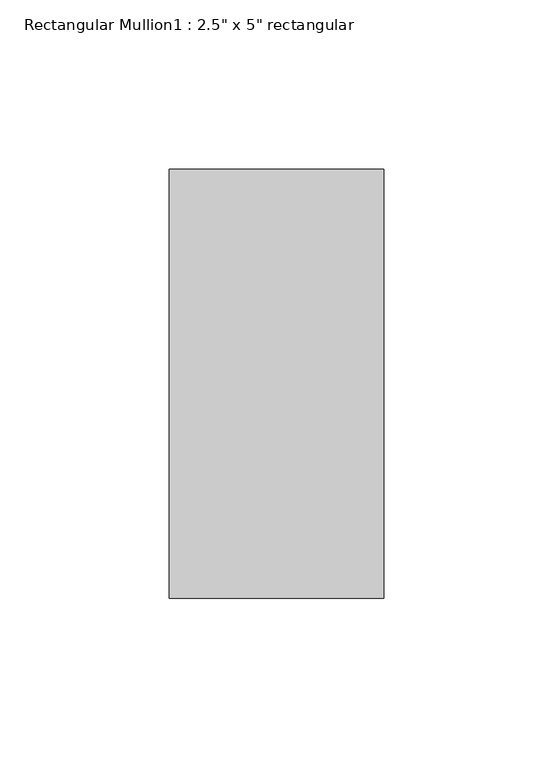
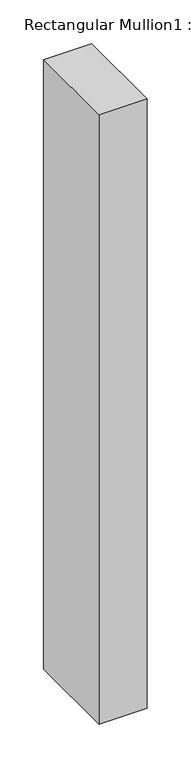
"""IFC4 building model written with IfcOpenShell, lengths in millimetres: member geometry."""

import ifcopenshell
import ifcopenshell.guid

model = None  # the IFC model being written
_history = None  # IfcOwnerHistory: only IFC2X3 demands one
_inside = {}  # id of a spatial element -> (the spatial element, [elements in it])
_under = {}  # id of a project, library or spatial element -> (it, [spatial elements below it])
_declared = {}  # id of a project -> (the project, [libraries it declares])
_typed = {}  # id of a type object -> (the type object, [elements of that type])
_made_of = {}  # id of a material, layer set ... -> (it, [elements and type objects made of it])


def new_model(schema):
    """Start an empty IFC model of exactly this schema.

    Asked for "IFC4X3", IfcOpenShell would pick the latest addendum, in which some entities
    have other attributes; the version numbers below select the first issue.
    IFC2X3 requires an IfcOwnerHistory on every rooted entity: one is made here for all.
    """
    global model, _history
    if schema == "IFC4X3":
        model = ifcopenshell.file(schema_version=(4, 3, 0, 0))
    else:
        model = ifcopenshell.file(schema=schema)
    _inside.clear()
    _under.clear()
    _declared.clear()
    _typed.clear()
    _made_of.clear()
    _history = None
    if model.schema == "IFC2X3":
        org = make("IfcOrganization", Name="unknown")
        user = make(
            "IfcPersonAndOrganization",
            ThePerson=make("IfcPerson", FamilyName="unknown"),
            TheOrganization=org,
        )
        app = make(
            "IfcApplication",
            ApplicationDeveloper=org,
            Version="unknown",
            ApplicationFullName="unknown",
            ApplicationIdentifier="unknown",
        )
        _history = make(
            "IfcOwnerHistory",
            OwningUser=user,
            OwningApplication=app,
            ChangeAction="ADDED",
            CreationDate=0,
        )
    return model


def make(cls, **values):
    """One entity of the class cls with the attributes given. An attribute that is None is left unset."""
    return model.create_entity(
        cls, **{name: value for name, value in values.items() if value is not None}
    )


def rooted(cls, **values):
    """An entity with a GlobalId (a new one), such as an element, a storey or a relation."""
    return make(cls, GlobalId=ifcopenshell.guid.new(), OwnerHistory=_history, **values)


def si_unit(unit_type, name, prefix=None):
    """IfcSIUnit, for example si_unit("LENGTHUNIT", "METRE", prefix="MILLI")."""
    return make("IfcSIUnit", UnitType=unit_type, Prefix=prefix, Name=name)


def assignment(units):
    """IfcUnitAssignment: the units of a project."""
    return None if units is None else make("IfcUnitAssignment", Units=units)


def point(xyz):
    """IfcCartesianPoint."""
    return None if xyz is None else make("IfcCartesianPoint", Coordinates=xyz)


def direction(xyz):
    """IfcDirection."""
    return None if xyz is None else make("IfcDirection", DirectionRatios=xyz)


def frame(location, z_axis=None, x_axis=None):
    """IfcAxis2Placement3D, a coordinate frame: its origin and axes. An axis left out is left unset."""
    return make(
        "IfcAxis2Placement3D",
        Location=point(location),
        Axis=direction(z_axis),
        RefDirection=direction(x_axis),
    )


def origin():
    """The frame at (0, 0, 0) with its axes left unset."""
    return frame((0.0, 0.0, 0.0))


def place(relative_to, where):
    """IfcLocalPlacement: puts the frame where relative to a parent placement (None: the world)."""
    return make(
        "IfcLocalPlacement", PlacementRelTo=relative_to, RelativePlacement=where
    )


def context(
    kind, dimensions, precision=None, world=None, true_north=None, identifier=None
):
    """IfcGeometricRepresentationContext, for example the 3D "Model" context."""
    return make(
        "IfcGeometricRepresentationContext",
        ContextIdentifier=identifier,
        ContextType=kind,
        CoordinateSpaceDimension=dimensions,
        Precision=precision,
        WorldCoordinateSystem=world,
        TrueNorth=true_north,
    )


def project(units=None, contexts=None):
    """IfcProject with its units and contexts."""
    return rooted(
        "IfcProject",
        Name="project",
        RepresentationContexts=contexts,
        UnitsInContext=assignment(units),
    )


def spatial(cls, under=None, at=None, **own):
    """A site, building, storey or space (cls), placed at a placement, below another one or the project."""
    s = rooted(cls, ObjectPlacement=at, **own)
    if under is not None:
        _under.setdefault(under.id(), (under, []))[1].append(s)
    return s


def polyline(points):
    """IfcPolyline through the points."""
    return make("IfcPolyline", Points=[point(p) for p in points])


def outline(outer, holes=None, kind="AREA"):
    """IfcArbitraryClosedProfileDef: a profile drawn as a closed curve; with holes, ...WithVoids."""
    if holes is None:
        return make("IfcArbitraryClosedProfileDef", ProfileType=kind, OuterCurve=outer)
    return make(
        "IfcArbitraryProfileDefWithVoids",
        ProfileType=kind,
        OuterCurve=outer,
        InnerCurves=holes,
    )


def extrude(swept, where, along, depth):
    """IfcExtrudedAreaSolid: the profile swept, set in the frame where, extruded along a direction by depth."""
    return make(
        "IfcExtrudedAreaSolid",
        SweptArea=swept,
        Position=where,
        ExtrudedDirection=direction(along),
        Depth=depth,
    )


def shape(context_of_items, identifier, shape_type, items):
    """IfcShapeRepresentation: the items that make up one representation, for example the "Body"."""
    return make(
        "IfcShapeRepresentation",
        ContextOfItems=context_of_items,
        RepresentationIdentifier=identifier,
        RepresentationType=shape_type,
        Items=items,
    )


def source(mapping_origin, context_of_items, identifier, shape_type, items):
    """IfcRepresentationMap: a shape defined once, which mapped items show again and again."""
    return make(
        "IfcRepresentationMap",
        MappingOrigin=mapping_origin,
        MappedRepresentation=shape(context_of_items, identifier, shape_type, items),
    )


def transform(
    local_origin,
    x_axis=None,
    y_axis=None,
    z_axis=None,
    scale=None,
    scale2=None,
    scale3=None,
    uniform=True,
):
    """IfcCartesianTransformationOperator3D, or its non-uniform kind. x_axis, y_axis, z_axis: its Axis1, 2, 3."""
    if uniform:
        return make(
            "IfcCartesianTransformationOperator3D",
            Axis1=direction(x_axis),
            Axis2=direction(y_axis),
            LocalOrigin=point(local_origin),
            Scale=scale,
            Axis3=direction(z_axis),
        )
    return make(
        "IfcCartesianTransformationOperator3DnonUniform",
        Axis1=direction(x_axis),
        Axis2=direction(y_axis),
        LocalOrigin=point(local_origin),
        Scale=scale,
        Axis3=direction(z_axis),
        Scale2=scale2,
        Scale3=scale3,
    )


def mapped(mapping_source, mapping_target):
    """IfcMappedItem: shows the shape of a source again, moved by a transform."""
    return make(
        "IfcMappedItem", MappingSource=mapping_source, MappingTarget=mapping_target
    )


def made_of(thing, what):
    """Note that an element or type object is made of a material, layer set ...; save() writes the relation."""
    if what is not None:
        _made_of.setdefault(what.id(), (what, []))[1].append(thing)
    return thing


def element(
    cls,
    number,
    at=None,
    inside=None,
    cuts=None,
    type_object=None,
    material=None,
    context=None,
    identifier="Body",
    shape_type=None,
    held_by="IfcProductDefinitionShape",
    body=None,
    shapes=None,
    **own,
):
    """One element of the class cls, such as IfcWall. Its Tag is "e" and its number.

    at: its placement. inside: the storey or other place that contains it. cuts: it is an
    opening in that element (IfcRelVoidsElement). A single representation is given by context,
    identifier, shape_type and body (its items); several are given by shapes. held_by: the class
    of the entity that holds the representations. save() writes the other relations.
    """
    e = rooted(cls, Tag="e%d" % number, ObjectPlacement=at, **own)
    if body is not None:
        shapes = [shape(context, identifier, shape_type, body)]
    if shapes is not None:
        e.Representation = make(held_by, Representations=shapes)
    if inside is not None:
        _inside.setdefault(inside.id(), (inside, []))[1].append(e)
    if cuts is not None:
        rooted(
            "IfcRelVoidsElement", RelatingBuildingElement=cuts, RelatedOpeningElement=e
        )
    if type_object is not None:
        _typed.setdefault(type_object.id(), (type_object, []))[1].append(e)
    return made_of(e, material)


def aggregate(whole, parts):
    """IfcRelAggregates: a whole, such as a stair, and the parts it consists of."""
    return rooted("IfcRelAggregates", RelatingObject=whole, RelatedObjects=parts)


def save(model, path):
    """Write the relations noted so far, then the file.

    IfcRelAggregates (storeys below a building ...), IfcRelContainedInSpatialStructure (elements
    in a storey), IfcRelDefinesByType, IfcRelAssociatesMaterial and IfcRelDeclares: one each for
    every whole, place, type object, material and project.
    """
    for whole, parts in _under.values():
        aggregate(whole, parts)
    for where, things in _inside.values():
        rooted(
            "IfcRelContainedInSpatialStructure",
            RelatedElements=things,
            RelatingStructure=where,
        )
    for kind, things in _typed.values():
        rooted("IfcRelDefinesByType", RelatedObjects=things, RelatingType=kind)
    for what, things in _made_of.values():
        rooted("IfcRelAssociatesMaterial", RelatedObjects=things, RelatingMaterial=what)
    for by, libraries in _declared.values():
        rooted("IfcRelDeclares", RelatingContext=by, RelatedDefinitions=libraries)
    model.write(path)


def member_d2e7e466(model_context):
    return source(origin(), model_context, "Body", "SweptSolid", [
        extrude(outline(polyline([(0.0, 63.5), (0.0, -63.5), (-63.5, -63.5), (-63.5, 63.5), (0.0, 63.5)])), frame((0.0, 0.0, -850.9), z_axis=(0.0, 0.0, 1.0), x_axis=(1.0, 0.0, 0.0)), (0.0, 0.0, 1.0), 850.9),
    ])


if __name__ == "__main__":
    model = new_model("IFC4")
    model_context = context("Model", 3, world=origin())
    ifc_project = project(units=[si_unit("LENGTHUNIT", "METRE", prefix="MILLI")], contexts=[model_context])
    site = spatial("IfcSite", under=ifc_project)
    building = spatial("IfcBuilding", under=site)
    placement = place(None, origin())
    member_shape = member_d2e7e466(model_context)
    element("IfcMember", 1, ObjectType="Rectangular Mullion1 : 2.5\" x 5\" rectangular", at=placement, inside=building, context=model_context, shape_type="MappedRepresentation", body=[
        mapped(member_shape, transform((0.0, 0.0, 0.0), x_axis=(1.0, 0.0, 0.0), y_axis=(0.0, 1.0, 0.0), z_axis=(0.0, 0.0, 1.0))),
    ])
    save(model, "model.ifc")

# Revit data of these elements
# Type "Rectangular Mullion1 : 2.5\" x 5\" rectangular"
#   built-in parameter 1007304 = 0.416667 (stored number, unit not read)
#   built-in parameter 1007301 = 0.104167 (stored number, unit not read)
#   built-in parameter 1007300 = 0.104167 (stored number, unit not read)
# Element 1 (IfcMember, "Rectangular Mullion1 : 2.5\" x 5\" rectangular")
#   Materials on its faces: "support-frame"
# Materials
#   "support-frame": class "Unassigned", colour RGB 233 233 233, transparency 0, Cost = 0
